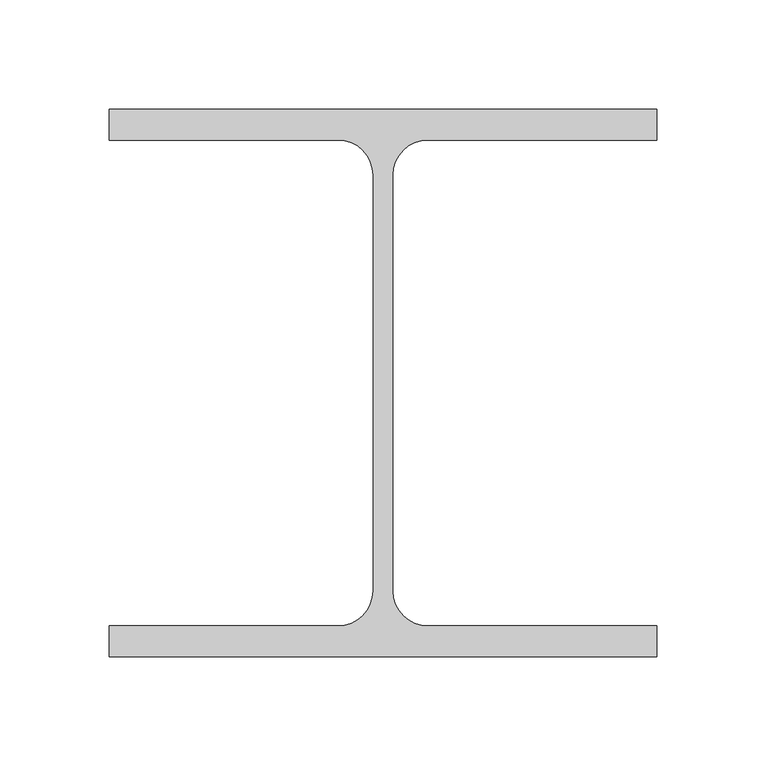
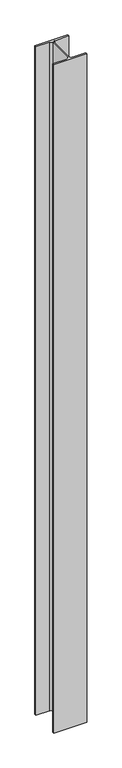
"""IFC4 building model written with IfcOpenShell, lengths in millimetres: column geometry, 0912_Steel Column_H_KSD3502 : H_SC_ASC_H-250x250x9x14."""

from ifc_helpers import new_model, si_unit, point, frame, frame_2d, origin, place, context, project, spatial, polyline, circle_curve, trimmed, segment, composite_curve, outline, extrude, source, transform, mapped, element, save


def column_c81c4db5(model_context):
    return source(origin(), model_context, "Body", "SweptSolid", [
        extrude(outline(composite_curve([segment(polyline([(125.0, 125.0), (125.0, 111.0), (20.5, 111.0)]), True, "CONTINUOUS"), segment(trimmed(circle_curve(frame_2d((20.5, 95.0)), 16.0), [point((20.5, 111.0))], [point((4.5, 95.0))], True, "CARTESIAN"), True, "CONTINUOUS"), segment(polyline([(4.5, 95.0), (4.5, -95.0)]), True, "CONTINUOUS"), segment(trimmed(circle_curve(frame_2d((20.5, -95.0)), 16.0), [point((4.5, -95.0))], [point((20.5, -111.0))], True, "CARTESIAN"), True, "CONTINUOUS"), segment(polyline([(20.5, -111.0), (125.0, -111.0), (125.0, -125.0), (-125.0, -125.0), (-125.0, -111.0), (-20.5, -111.0)]), True, "CONTINUOUS"), segment(trimmed(circle_curve(frame_2d((-20.5, -95.0)), 16.0), [point((-20.5, -111.0))], [point((-4.5, -95.0))], True, "CARTESIAN"), True, "CONTINUOUS"), segment(polyline([(-4.5, -95.0), (-4.5, 95.0)]), True, "CONTINUOUS"), segment(trimmed(circle_curve(frame_2d((-20.5, 95.0)), 16.0), [point((-4.5, 95.0))], [point((-20.5, 111.0))], True, "CARTESIAN"), True, "CONTINUOUS"), segment(polyline([(-20.5, 111.0), (-125.0, 111.0), (-125.0, 125.0), (125.0, 125.0)]), True, "CONTINUOUS")], self_intersect=False)), frame((0.0, 0.0, 599.9720055), z_axis=(0.0, 0.0, 1.0), x_axis=(1.0, 0.0, 0.0)), (0.0, 0.0, 1.0), 5350.0),
    ])


if __name__ == "__main__":
    model = new_model("IFC4")
    model_context = context("Model", 3, world=origin())
    ifc_project = project(units=[si_unit("LENGTHUNIT", "METRE", prefix="MILLI")], contexts=[model_context])
    site = spatial("IfcSite", under=ifc_project)
    building = spatial("IfcBuilding", under=site)
    placement = place(None, origin())
    column_shape = column_c81c4db5(model_context)
    element("IfcColumn", 1, ObjectType="0912_Steel Column_H_KSD3502 : H_SC_ASC_H-250x250x9x14", at=placement, inside=building, context=model_context, shape_type="MappedRepresentation", body=[
        mapped(column_shape, transform((0.0, 0.0, 0.0), x_axis=(1.0, 0.0, 0.0), y_axis=(0.0, 1.0, 0.0), z_axis=(0.0, 0.0, 1.0))),
    ])
    save(model, "model.ifc")

# Revit data of these elements
# Type "0912_Steel Column_H_KSD3502 : H_SC_ASC_H-250x250x9x14"
#   H_WM Code_1 = "S01AA002-00001 | Main Steel Structure Fabrication Work | Shelter/Building | Medium Steel - Standard (90KG/M>Weight≥30KG/M) | Material: (   )"
#   H_WM Code_2 = "S03AA028-00001 | Main Steel Structure Erection Work | Shelter/Building | Medium Steel (90KG/M>Weight≥30KG/M) | Material: (   )"
#   H_WM Code_3 = "S01AA010-00001 | Main Steel Structure Fabrication Work | Shelter/Building | Steel Painting/Coating | for Non-Fireproofed Steel Surface, Surface Preparation, Primer, Second & Final Coat | Material: (   )"
#   H_Q'ty Cal Type Tag = "SC-Q2"
#   Width = 25.0 cm
#   Web Thickness = 0.9 cm
#   Web Fillet = 1.6 cm
#   Warping Constant = 507646.0 cm⁶
#   Torsional Moment of Inertia = 51.4681 cm⁴
#   Section Area = 92.18 cm²
#   Plastic Modulus weak axis = 444.0 cm³
#   Plastic Modulus strong axis = 960.0 cm³
#   Perimeter = 1.46 m²/m
#   Nominal Weight = 72.40 kgf/m
#   Moment of Inertia weak axis = 3650.00 cm⁴
#   Moment of Inertia strong axis = 10800.00 cm⁴
#   Height = 25.0 cm
#   Flange Thickness = 1.4 cm
#   Elastic Modulus weak axis = 292.0 cm³
#   Elastic Modulus strong axis = 867.0 cm³
#   Centroid Vertical = 12.5 cm
#   Centroid Horizontal = 12.5 cm
#   Structural Material [instance default] = Steel, 45-345
#   Section Name Key = ""
#   Bolt Spacing = 0
#   Assembly Code = ""
# Element 1 (IfcColumn, "0912_Steel Column_H_KSD3502 : H_SC_ASC_H-250x250x9x14")
#   Structural Material = A03AD029-00005_Anchor Bolt (Installation only)_M24
#   Materials on its faces: "A03AD029-00005_Anchor Bolt (Installation only)_M24"
# Materials
#   "Steel, 45-345": class "Metal", colour RGB 189 187 185, transparency 0, Description = "Steel 345 MPa", Cost = 0
#   "A03AD029-00005_Anchor Bolt (Installation only)_M24": class "Unassigned", colour RGB 84 83 81, transparency 0, Cost = 0
